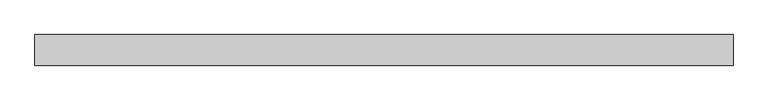
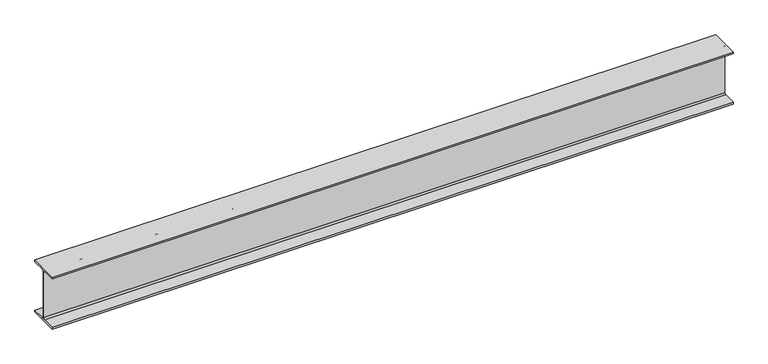
"""IFC4 building model written with IfcOpenShell, lengths in millimetres: beam geometry, Old_Steel Beam_H-KSD3502 : H_SB_ASB_H-200×200x8x12."""

from ifc_helpers import new_model, si_unit, point, frame, frame_2d, origin, place, context, project, spatial, polyline, circle_curve, trimmed, segment, composite_curve, outline, extrude, source, transform, mapped, element, save


def beam_cb92c45f(model_context):
    return source(origin(), model_context, "Body", "SweptSolid", [
        extrude(outline(composite_curve([segment(polyline([(82.5, -141.5), (82.5, -151.7), (-82.5, -151.7), (-82.5, -141.5), (-11.9, -141.5)]), True, "CONTINUOUS"), segment(trimmed(circle_curve(frame_2d((-11.9, -132.6)), 8.9), [point((-11.9, -141.5))], [point((-3.0, -132.6))], True, "CARTESIAN"), True, "CONTINUOUS"), segment(polyline([(-3.0, -132.6), (-3.0, 132.6)]), True, "CONTINUOUS"), segment(trimmed(circle_curve(frame_2d((-11.9, 132.6)), 8.9), [point((-3.0, 132.6))], [point((-11.9, 141.5))], True, "CARTESIAN"), True, "CONTINUOUS"), segment(polyline([(-11.9, 141.5), (-82.5, 141.5), (-82.5, 151.7), (82.5, 151.7), (82.5, 141.5), (11.9, 141.5)]), True, "CONTINUOUS"), segment(trimmed(circle_curve(frame_2d((11.9, 132.6)), 8.9), [point((11.9, 141.5))], [point((3.0, 132.6))], True, "CARTESIAN"), True, "CONTINUOUS"), segment(polyline([(3.0, 132.6), (3.0, -132.6)]), True, "CONTINUOUS"), segment(trimmed(circle_curve(frame_2d((11.9, -132.6)), 8.9), [point((3.0, -132.6))], [point((11.9, -141.5))], True, "CARTESIAN"), True, "CONTINUOUS"), segment(polyline([(11.9, -141.5), (82.5, -141.5)]), True, "CONTINUOUS")], self_intersect=False)), frame((-1938.4214468, 0.0, 0.0), z_axis=(1.0, 0.0, 0.0), x_axis=(0.0, 1.0, 0.0)), (0.0, 0.0, 1.0), 3758.8913358),
    ])


if __name__ == "__main__":
    model = new_model("IFC4")
    model_context = context("Model", 3, world=origin())
    ifc_project = project(units=[si_unit("LENGTHUNIT", "METRE", prefix="MILLI")], contexts=[model_context])
    site = spatial("IfcSite", under=ifc_project)
    building = spatial("IfcBuilding", under=site)
    placement = place(None, origin())
    beam_shape = beam_cb92c45f(model_context)
    element("IfcBeam", 1, ObjectType="Old_Steel Beam_H-KSD3502 : H_SB_ASB_H-200×200x8x12", at=placement, inside=building, context=model_context, shape_type="MappedRepresentation", body=[
        mapped(beam_shape, transform((0.0, 0.0, 0.0), x_axis=(1.0, 0.0, 0.0), y_axis=(0.0, 1.0, 0.0), z_axis=(0.0, 0.0, 1.0))),
    ])
    save(model, "model.ifc")

# Revit data of these elements
# Type "Old_Steel Beam_H-KSD3502 : H_SB_ASB_H-200×200x8x12"
#   Width = 20.0 cm
#   Web Thickness = 0.8 cm
#   Web Fillet = 1.3 cm
#   Warping Constant = 141376.0 cm⁶
#   Torsional Moment of Inertia = 26.2485 cm⁴
#   Torsional Modulus = 1.0 cm³
#   Section Area = 63.53 cm²
#   Plastic Modulus weak axis = 244.0 cm³
#   Plastic Modulus strong axis = 525.0 cm³
#   Perimeter = 1.16 m²/m
#   Nominal Weight = 49.90 kgf/m
#   Moment of Inertia weak axis = 1600.00 cm⁴
#   Moment of Inertia strong axis = 4720.00 cm⁴
#   Height = 20.0 cm
#   Flange Thickness = 1.2 cm
#   Elastic Modulus weak axis = 160.0 cm³
#   Elastic Modulus strong axis = 472.0 cm³
#   Centroid Vertical = 10.0 cm
#   Centroid Horizontal = 10.0 cm
#   Length [instance default] = 1.5240 m
#   Structural Material [instance default] = Steel, 45-345
#   Assembly Code = ""
# Element 1 (IfcBeam, "Old_Steel Beam_H-KSD3502 : H_SB_ASB_H-200×200x8x12")
#   Structural Material = none
# Materials
#   "Steel, 45-345": class "Metal", colour RGB 189 187 185, transparency 0, Description = "Steel 345 MPa", Cost = 0
